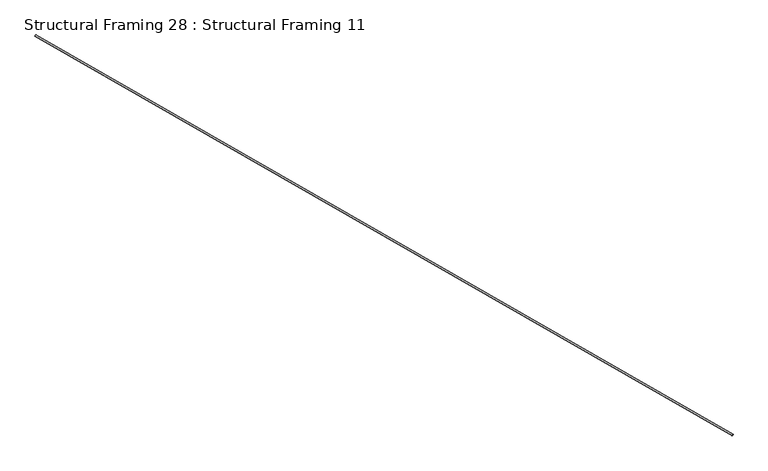
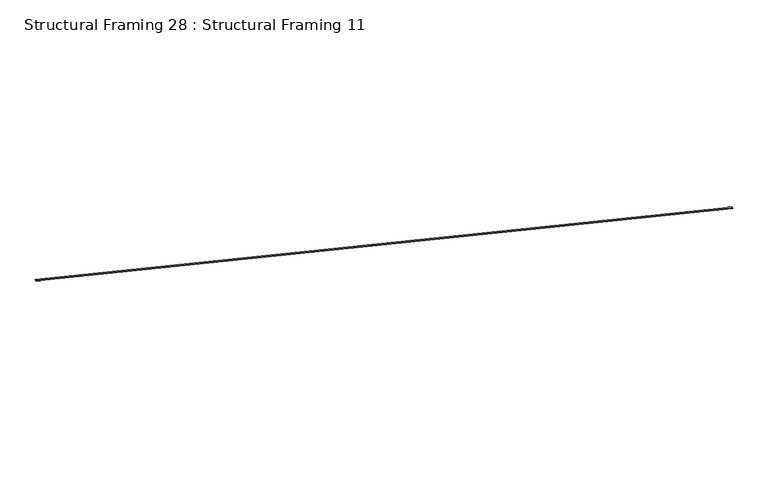
"""IFC4 building model written with IfcOpenShell, lengths in millimetres: beam geometry, Structural Framing 28 : Structural Framing 11."""

from ifc_helpers import new_model, si_unit, point, frame, origin, origin_2d, place, context, project, spatial, circle_curve, trimmed, segment, composite_curve, outline, extrude, source, transform, mapped, element, save


def structural_framing_28_structural_framing_11_3ea5cd18(model_context):
    return source(origin(), model_context, "Body", "SweptSolid", [
        extrude(outline(composite_curve([segment(trimmed(circle_curve(origin_2d(), 6.35), [point((0.0, -6.35))], [point((0.0, 6.35))], False, "CARTESIAN"), True, "CONTINUOUS"), segment(trimmed(circle_curve(origin_2d(), 6.35), [point((0.0, 6.35))], [point((0.0, -6.35))], False, "CARTESIAN"), True, "CONTINUOUS")], self_intersect=False)), frame((23230.1665052, 10045.6198795, 4934.1500933), z_axis=(0.8608596592499212, -0.49364969439625495, 0.12341242359906028), x_axis=(0.0, 0.24253562503632656, 0.9701425001453335)), (0.0, 0.0, 1.0), 5892.4476777),
    ])


if __name__ == "__main__":
    model = new_model("IFC4")
    model_context = context("Model", 3, world=origin())
    ifc_project = project(units=[si_unit("LENGTHUNIT", "METRE", prefix="MILLI")], contexts=[model_context])
    site = spatial("IfcSite", under=ifc_project)
    building = spatial("IfcBuilding", under=site)
    placement = place(None, origin())
    structural_framing_28_structural_framing_11_shape = structural_framing_28_structural_framing_11_3ea5cd18(model_context)
    element("IfcBeam", 1, ObjectType="Structural Framing 28 : Structural Framing 11", at=placement, inside=building, context=model_context, shape_type="MappedRepresentation", body=[
        mapped(structural_framing_28_structural_framing_11_shape, transform((0.0, 0.0, 0.0), x_axis=(1.0, 0.0, 0.0), y_axis=(0.0, 1.0, 0.0), z_axis=(0.0, 0.0, 1.0))),
    ])
    save(model, "model.ifc")

# Revit data of these elements
# Type "Structural Framing 28 : Structural Framing 11"
#   Structural Material [instance default] = EXISTING LATERAL BRACING (1/4" CABLE)
# Element 1 (IfcBeam, "Structural Framing 28 : Structural Framing 11")
#   Materials on its faces: "EXISTING LATERAL BRACING (1/4\" CABLE)"
# Materials
#   "EXISTING LATERAL BRACING (1/4\" CABLE)": class "Generic", colour RGB 120 120 120, transparency 0, Cost = 0
